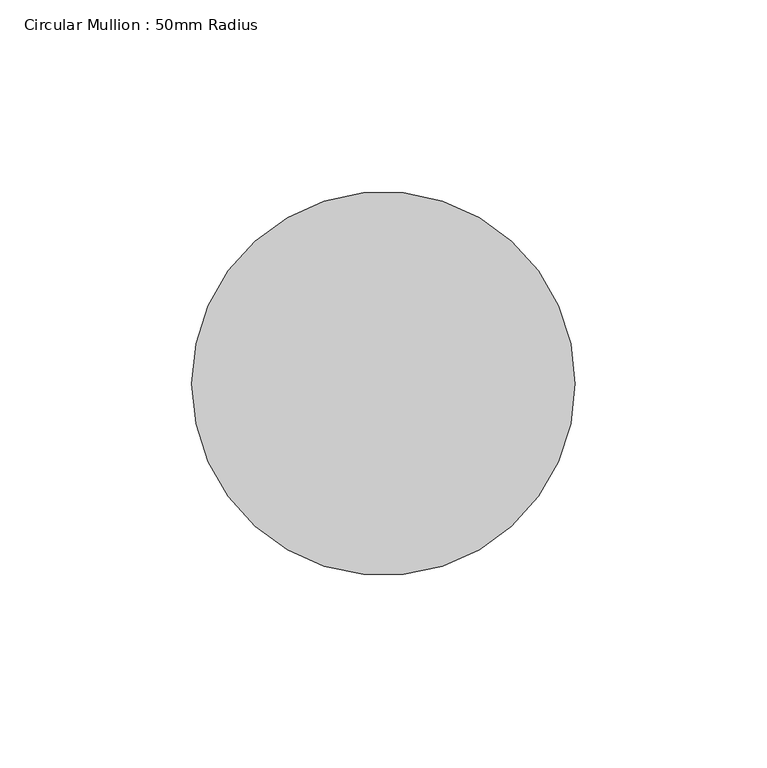
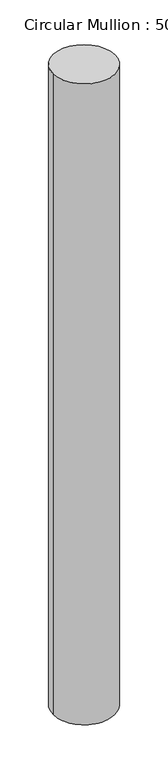
"""IFC4 building model written with IfcOpenShell, lengths in millimetres: member geometry, Circular Mullion : 50mm Radius."""

from ifc_helpers import new_model, si_unit, frame, origin, place, context, project, spatial, ellipse_curve, source, transform, mapped, element, save
from ifc_brep_helpers import plane_surface, cylinder_surface, advanced_brep


def circular_mullion_50mm_radius_8d295625(model_context):
    return source(origin(), model_context, "Body", "AdvancedBrep", [
        advanced_brep(
        [(-100.0, 0.0, 1.7650114), (0.0, 0.0, 0.0), (0.0, 0.0, -1094.6825184), (-100.0, 0.0, -1096.3690318)],
        [
            (0, 1, ellipse_curve(frame((-50.0, 0.0, 0.8825057), z_axis=(-0.01764332631957105, -0.021393878317499088, -0.9996154335577845), x_axis=(-0.6359961507311636, -0.7711938221109275, 0.02773057866475636)), 50.0192357, 50.0)),
            (1, 2),
            (2, 3, ellipse_curve(frame((-50.0, 0.0, -1095.5257751), z_axis=(-0.016859212013722157, -0.020443079939543987, 0.9996488620775106), x_axis=(0.6360174193202606, 0.7712196118966747, 0.0264981612029637)), 50.0175631, 50.0)),
            (3, 0),
            (1, 0, ellipse_curve(frame((-50.0, 0.0, 0.8825057), z_axis=(-0.01764332631957105, -0.021393878317499088, -0.9996154335577845), x_axis=(-0.6359961507311636, -0.7711938221109275, 0.02773057866475636)), 50.0192357, 50.0)),
            (3, 2, ellipse_curve(frame((-50.0, 0.0, -1095.5257751), z_axis=(-0.016859212013722157, -0.020443079939543987, 0.9996488620775106), x_axis=(0.6360174193202606, 0.7712196118966747, 0.0264981612029637)), 50.0175631, 50.0)),
        ],
        [
            cylinder_surface(frame((-50.0, 0.0, 0.0), z_axis=(0.0, 0.0, 1.0), x_axis=(1.0, 0.0, 0.0)), 50.0),
            plane_surface(frame((-235.1503079, 193.9262043, 0.0), z_axis=(0.017643326319571054, 0.02139387831749909, 0.9996154335577847), x_axis=(0.635996150731163, 0.7711938221109277, -0.02773057866476692))),
            plane_surface(frame((-235.1503079, 193.9262043, -1094.6825184), z_axis=(0.01685921201372216, 0.02044307993954399, -0.9996488620775108), x_axis=(0.6360174193202607, 0.7712196118966748, 0.02649816120296311))),
        ],
        [
            (0, [[1, 2, 3, 4]]),
            (0, [[5, -4, 6, -2]]),
            (1, [[-1, -5]]),
            (2, [[-6, -3]]),
        ],
    ),
    ])


if __name__ == "__main__":
    model = new_model("IFC4")
    model_context = context("Model", 3, world=origin())
    ifc_project = project(units=[si_unit("LENGTHUNIT", "METRE", prefix="MILLI")], contexts=[model_context])
    site = spatial("IfcSite", under=ifc_project)
    building = spatial("IfcBuilding", under=site)
    placement = place(None, origin())
    circular_mullion_50mm_radius_shape = circular_mullion_50mm_radius_8d295625(model_context)
    element("IfcMember", 1, ObjectType="Circular Mullion : 50mm Radius", at=placement, inside=building, context=model_context, shape_type="MappedRepresentation", body=[
        mapped(circular_mullion_50mm_radius_shape, transform((0.0, 0.0, 0.0), x_axis=(1.0, 0.0, 0.0), y_axis=(0.0, 1.0, 0.0), z_axis=(0.0, 0.0, 1.0))),
    ])
    save(model, "model.ifc")

# Revit data of these elements
# Type "Circular Mullion : 50mm Radius"
#   built-in parameter 1007350 = 0.164042 (stored number, unit not read)
# Element 1 (IfcMember, "Circular Mullion : 50mm Radius")
#   Materials on its faces: "Aluminium"
# Materials
#   "Aluminium": class "Metal", colour RGB 247 247 247, transparency 0, Description = "Aluminium 6061", Cost = 0
